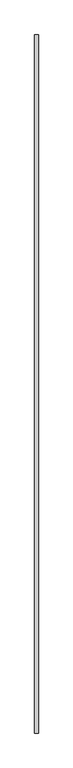
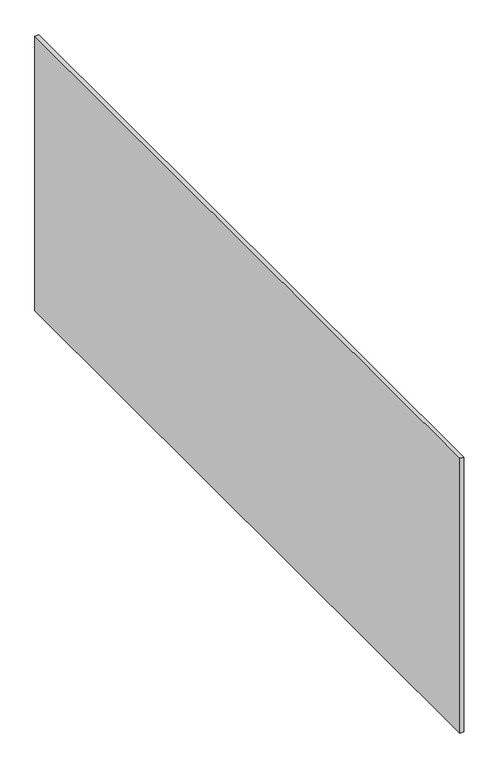
"""IFC4 building model written with IfcOpenShell, lengths in millimetres: proxy geometry, Inner panel:Inner panel:1:Inner panel:1 : Inner panel:Inner panel:300324:300043:Inner panel:1:Inner panel:1 : Inner panel:Inner panel:300324:300043 : Inner panel:Inner panel:1:Inner panel:1 : Inner panel:Inner panel:300324:300043:32 : Inner panel:Inner panel:1:Inner panel:1 : Inner panel:Inner panel:300324:300043:Inner panel:1:Inner panel:1 : Inner panel:Inner panel:300324:300043 : Inner panel:Inner panel:1:Inner panel:1 : Inner panel:Inner panel:300324:300043:300031."""

from ifc_helpers import new_model, si_unit, frame, origin, place, context, project, spatial, polyline, outline, extrude, source, transform, mapped, element, save


def generic_models_426c844a(model_context):
    return source(origin(), model_context, "Body", "SweptSolid", [
        extrude(outline(polyline([(579307.711724, -576279.7163841), (579320.4117239, -576279.7163841), (579320.4117239, -578718.1163841), (579307.711724, -578718.1163841), (579307.711724, -576279.7163841)])), frame((0.0, 0.0, 3978.2465087), z_axis=(0.0, 0.0, 1.0), x_axis=(1.0, 0.0, 0.0)), (0.0, 0.0, 1.0), 962.0534913),
    ])


if __name__ == "__main__":
    model = new_model("IFC4")
    model_context = context("Model", 3, world=origin())
    ifc_project = project(units=[si_unit("LENGTHUNIT", "METRE", prefix="MILLI")], contexts=[model_context])
    site = spatial("IfcSite", under=ifc_project)
    building = spatial("IfcBuilding", under=site)
    placement = place(None, origin())
    generic_models_shape = generic_models_426c844a(model_context)
    element("IfcBuildingElementProxy", 1, Name="Inner panel:Inner panel:1:Inner panel:1 : Inner panel:Inner panel:300324:300043:Inner panel:1:Inner panel:1 : Inner panel:Inner panel:300324:300043 : Inner panel:Inner panel:1:Inner panel:1 : Inner panel:Inner panel:300324:300043:32 : Inner panel:Inner panel:1:Inner panel:1 : Inner panel:Inner panel:300324:300043:Inner panel:1:Inner panel:1 : Inner panel:Inner panel:300324:300043 : Inner panel:Inner panel:1:Inner panel:1 : Inner panel:Inner panel:300324:300043:300031", ObjectType="Inner panel:Inner panel:1:Inner panel:1 : Inner panel:Inner panel:300324:300043:Inner panel:1:Inner panel:1 : Inner panel:Inner panel:300324:300043 : Inner panel:Inner panel:1:Inner panel:1 : Inner panel:Inner panel:300324:300043:32 : Inner panel:Inner panel:1:Inner panel:1 : Inner panel:Inner panel:300324:300043:Inner panel:1:Inner panel:1 : Inner panel:Inner panel:300324:300043 : Inner panel:Inner panel:1:Inner panel:1 : Inner panel:Inner panel:300324:300043:300031", at=placement, inside=building, context=model_context, shape_type="MappedRepresentation", body=[
        mapped(generic_models_shape, transform((0.0, 0.0, 0.0), x_axis=(1.0, 0.0, 0.0), y_axis=(0.0, 1.0, 0.0), z_axis=(0.0, 0.0, 1.0))),
    ])
    save(model, "model.ifc")

# Revit data of these elements
# Type "Inner panel:Inner panel:1:Inner panel:1 : Inner panel:Inner panel:300324:300043:Inner panel:1:Inner panel:1 : Inner panel:Inner panel:300324:300043 : Inner panel:Inner panel:1:Inner panel:1 : Inner panel:Inner panel:300324:300043:32 : Inner panel:Inner panel:1:Inner panel:1 : Inner panel:Inner panel:300324:300043:Inner panel:1:Inner panel:1 : Inner panel:Inner panel:300324:300043 : Inner panel:Inner panel:1:Inner panel:1 : Inner panel:Inner panel:300324:300043:300031"
#   NameOverride = "Inner panel:Inner panel:1:Inner panel:1 : Inner panel:Inner panel:300324:300043:Inner panel:1:Inner panel:1 : Inner panel:Inner panel:300324:300043 : Inner panel:Inner panel:1:Inner panel:1 : Inner panel:Inner panel:300324:300043:300031"
#   ObjectTypeOverride = "Inner panel:1:Inner panel:1 : Inner panel:Inner panel:300324:300043 : Inner panel:Inner panel:1:Inner panel:1 : Inner panel:Inner panel:300324:300043"
#   Reference = "Inner panel"
#   Tag = "300031"
# Element 1 (IfcBuildingElementProxy, "Inner panel:Inner panel:1:Inner panel:1 : Inner panel:Inner panel:300324:300043:Inner panel:1:Inner panel:1 : Inner panel:Inner panel:300324:300043 : Inner panel:Inner panel:1:Inner panel:1 : Inner panel:Inner panel:300324:300043:32 : Inner panel:Inner panel:1:Inner panel:1 : Inner panel:Inner panel:300324:300043:Inner panel:1:Inner panel:1 : Inner panel:Inner panel:300324:300043 : Inner panel:Inner panel:1:Inner panel:1 : Inner panel:Inner panel:300324:300043:300031")
#   Materials on its faces: "1/2\" EXTERIOR GRADE FIRE RETARDANT CDX PLYWOOD"
# Materials
#   "1/2\" EXTERIOR GRADE FIRE RETARDANT CDX PLYWOOD": class "Unassigned", colour RGB 196 177 123, transparency 0, Cost = 0
